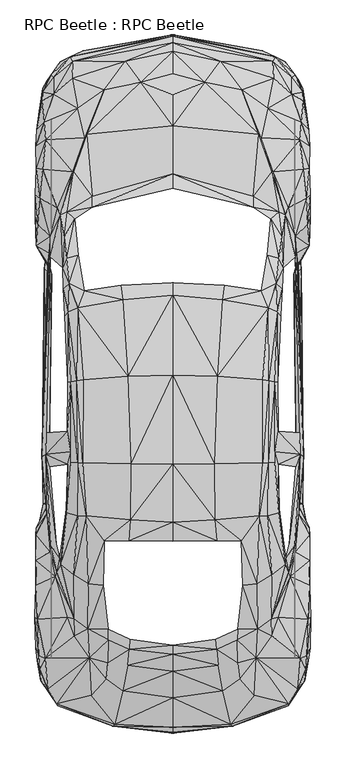
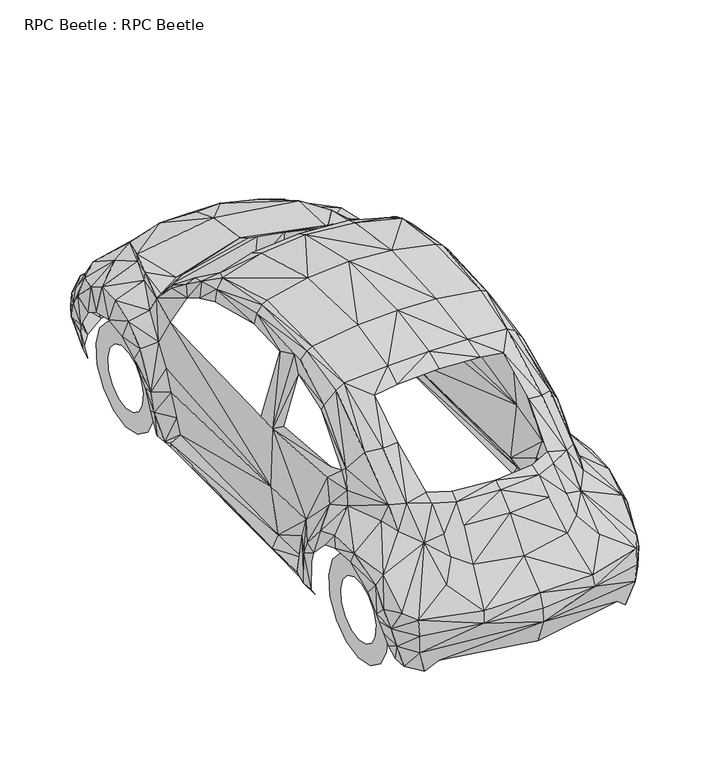
"""IFC4 building model written with IfcOpenShell, lengths in millimetres: proxy geometry, RPC Beetle : RPC Beetle."""

from ifc_helpers import new_model, si_unit, origin, place, context, project, spatial, triangles, source, transform, mapped, element, save


def rpc_beetle_rpc_beetle_e6dad58a(model_context):
    return source(origin(), model_context, "Body", "Tessellation", [
        triangles([(0.0, -748.5645555, 521.3897593), (0.0, -720.145796, 603.6245653), (0.0, -696.6751356, 283.1364967), (0.0, -552.6985313, 738.4055826), (0.0, -753.24988, 438.4543419), (0.0, -253.6668202, 1039.7142986), (0.0, -401.1027337, 921.397756), (0.0, -304.8118089, 1012.2589251), (0.0, 339.3171518, 1395.7149525), (0.0, 448.6132421, 1442.130724), (0.0, 778.0780157, 1504.0475842), (0.0, 1285.0174942, 1509.4774853), (0.0, 1741.0748314, 1402.3269035), (0.0, 2430.9628086, 967.2005562), (0.0, 3130.0025528, 632.0433249), (0.0, 3001.4394699, 771.5097393), (0.0, 2704.2468544, 928.754211), (0.0, 3164.2013374, 220.1686106), (0.0, 2883.1667473, 858.7363918), (0.0, 3222.5277191, 395.8043289), (0.0, 3179.0018875, 555.7637512), (0.0, 3213.9451035, 530.2788242), (-338.1786312, -715.5042189, 523.0099365), (-331.0411308, -702.1487114, 593.4656287), (-244.7339716, -218.0229748, 1034.0655882), (-248.9814594, -275.9551764, 1002.9319508), (-257.7391552, -368.1737844, 911.8518997), (-249.0690268, 342.8202084, 1381.001897), (-285.2383307, -511.5373446, 760.4312004), (-240.1361781, 460.085834, 1426.5857426), (-236.4579324, 780.8804609, 1493.4070999), (-652.4925127, -590.2252742, 370.4945729), (-540.0874552, -593.3342777, 283.4430006), (-181.240627, 2954.2792671, 806.3215679), (-253.1851454, 1278.5806778, 1496.1656525), (-379.8652946, -444.3657907, 798.2645016), (-370.9324459, -353.3294506, 889.169418), (-367.9986134, -222.226679, 1003.4574274), (-368.3927027, -160.7038173, 1036.6928988), (-390.1556185, 342.8640284, 1359.0200993), (-282.5672364, 1713.2691158, 1399.3055763), (-397.3369025, 87.4894363, 1215.350017), (-463.1072702, -537.7666666, 704.819842), (-271.488752, 3072.3331078, 662.6953056), (-475.7621301, -323.0715955, 849.8473269), (-463.7202779, 3085.9075699, 214.2571618), (-482.2428391, 95.7654664, 1203.3957321), (-485.0452844, -159.3025947, 1005.0776047), (-568.725133, 3071.5011818, 546.7432989), (-493.54026, 483.2499724, 1391.2922573), (-583.2629085, 3099.3942467, 522.0465869), (-510.267473, 3132.2794487, 369.399836), (-391.8633631, 2911.6292542, 782.7633402), (-656.3459112, -597.8445039, 480.0971852), (-660.2431297, -584.8393021, 576.2567591), (-562.2882076, -200.069692, 879.711129), (-560.0550227, -101.4579695, 987.1680874), (-512.4569106, 786.1788294, 1448.4362984), (-541.7951998, 484.7825824, 1359.8520252), (-563.9959886, 148.5744068, 1172.3059147), (-608.4850971, -561.2372907, 218.460866), (-511.2746063, 1258.5255066, 1456.1868427), (-542.4082438, 784.6900394, 1430.6581684), (-458.8597824, 2304.063723, 949.0283369), (-601.0410384, -92.7440574, 893.1979511), (-503.7429803, 1765.2899231, 1320.9679161), (-546.0426876, 1253.0081108, 1441.51768), (-603.0115213, 501.1594534, 1278.5806778), (-580.1539412, 788.8937799, 1378.7250011), (-607.2152255, 519.8571493, 1235.1424862), (-601.2599931, 965.2738569, 1337.0383015), (-712.482819, -503.0861526, 590.4880125), (-542.6709821, 1670.0499516, 1361.1657532), (-490.6064275, 2657.8746849, 893.5044731), (-599.6398158, 778.0780157, 1307.3059593), (-598.0634222, 1243.7249565, 1343.7817852), (-639.5749146, 208.1267766, 1062.4843477), (-680.4296156, -470.200987, 218.6798025), (-538.4672779, 1966.7170177, 1180.5819357), (-580.9859035, 1248.2351463, 1401.7577522), (-644.5230137, 243.2889472, 1028.2854904), (-502.3417577, 2635.8053925, 866.0052795), (-660.7247864, 162.2364272, 955.2462713), (-690.2382465, -396.5925076, 226.8244725), (-559.1354568, 2175.0189835, 1011.1642244), (-670.1830753, 140.867628, 872.7049433), (-662.476351, 324.2976834, 1009.4564798), (-615.0971935, 1623.4589001, 1262.1161304), (-594.647933, 1646.0976345, 1321.2744381), (-589.4370955, 1809.603788, 1269.4287655), (-728.8159063, -481.9801008, 373.2094508), (-751.5859554, -454.4371236, 476.5503087), (-694.0478251, 315.3210511, 957.7860146), (-726.5826851, -327.3190833, 735.5593174), (-622.9353052, 1777.2441353, 1192.7989225), (-564.6528162, 2445.7196114, 934.1402195), (-731.7935589, -393.8776297, 324.1225488), (-571.0021379, 2444.2743507, 884.1775715), (-698.6456549, 279.8523585, 807.6352232), (-604.281393, 1949.7708138, 1170.4667828), (-587.422829, 3013.0873055, 200.1134757), (-690.9388578, 574.2424925, 283.6181534), (-750.2284801, -381.0038152, 396.9865969), (-627.533135, 1896.2612892, 1124.7078026), (-602.486081, 2215.5670898, 949.1596516), (-619.4322487, 2072.8166462, 1075.2705585), (-710.4685524, 549.6333478, 448.6132421), (-764.7225082, -360.3356363, 467.5298927), (-699.5214008, 762.6206743, 1015.4992796), (-763.3212856, -313.2191809, 670.9275066), (-757.8477098, -390.9437971, 564.6528162), (-717.4746655, 496.2989579, 583.5694304), (-722.7292866, 461.2243546, 180.9779068), (-717.6498728, 554.4500959, 179.883188), (-771.4659193, -341.8130751, 511.011868), (-573.9359705, 2975.4727409, 682.6190168), (-730.7864256, 375.880545, 185.1815928), (-541.1821558, 2805.3982384, 782.9385475), (-639.7501219, 2198.4457512, 944.2553724), (-738.9310593, 551.5600471, 222.4018318), (-781.5810722, -268.773856, 609.2294921), (-772.2979179, -106.055763, 755.9210106), (-721.7221533, 957.7422672, 967.0254215), (-703.3309793, 810.1311464, 292.3320837), (-724.8311932, 835.0468494, 964.354291), (-757.7601425, 370.5383566, 225.4670335), (-785.3469034, -89.941594, 695.4928677), (-779.654373, 80.9211599, 675.5690838), (-779.391671, 89.5037119, 754.6511026), (-760.3874531, 444.1030523, 223.1462268), (-778.0780157, 192.1001749, 630.9048042), (-658.6229525, 2237.154871, 849.7597595), (-770.9404427, 345.4913389, 426.193535), (-774.1807972, 315.1458801, 501.68493), (-781.1869829, 232.2542464, 695.886957), (-719.22623, 810.0873991, 185.8384204), (-689.8879045, 1858.8658974, 293.9084591), (-696.6751356, 1958.8788334, 956.4286119), (-779.7419403, 377.3693713, 532.3806581), (-778.121763, 416.9979481, 439.7241772), (-745.4993357, 819.5895081, 613.6521509), (-677.7147377, 2884.8305992, 670.6209846), (-697.5509542, 2077.4143307, 756.8843239), (-639.6187346, 3069.1803932, 391.6881921), (-713.0082956, 1918.243087, 536.7157496), (-718.1752768, 1909.8794987, 192.9759572), (-705.1701113, 1981.9554771, 648.2888449), (-730.7864256, 1891.0943081, 233.348947), (-673.9927265, 2907.8634956, 198.6684513), (-726.8892071, 2038.9242382, 189.9545391), (-721.634586, 1973.3728615, 189.9545391), (-678.1963943, 2982.566494, 540.5253282), (-699.6089682, 2815.6885986, 206.2000773), (-696.3686136, 2991.5871643, 517.4050097), (-723.6488525, 2624.6831062, 787.5801247), (-699.0834915, 1882.4679451, 390.3745368), (-764.8976429, 2042.1645927, 362.5688576), (-741.7773245, 2457.6738235, 808.6861765), (-716.1610102, 2965.1387787, 449.5328081), (-766.4302528, 2001.1348297, 376.5811563), (-731.5746042, 2724.4334129, 727.6336384), (-771.1593973, 2084.5957237, 482.2428391), (-759.1175451, 2291.4088268, 780.0922823), (-769.0137434, 2143.3161221, 699.0397442), (-777.5525391, 2022.8538528, 494.8101316), (-742.4779358, 2846.8660561, 601.8730371), (-782.1065489, 2185.659613, 616.4545961), (-739.5441032, 2918.4163399, 427.3758393), (-741.1204605, 2896.5223274, 519.8133657), (-750.4036148, 2804.4349251, 398.0813338), (-782.2378635, 2313.1717426, 680.7361376), (-778.0780157, 2462.7970573, 693.5223484), (-759.9057238, 2786.6130478, 455.2253386), (-774.1807972, 2682.8342079, 602.6612157), (-780.3549843, 2589.4335136, 666.3297495), (-742.6093231, 809.1240131, 220.3875652), (0.0, 2349.0782719, 1011.1642244), (-458.8597824, 2239.9573162, 1006.6102146), (0.0, 1812.0122166, 1368.2157589), (-293.9522428, 1795.8104439, 1359.1514866), (-580.2415086, 849.7160122, 1381.7900757), (338.1786312, -715.5042189, 523.0099365), (331.0411308, -702.1487114, 593.4656287), (244.7339716, -218.0229748, 1034.0655882), (248.9814594, -275.9551764, 1002.9319508), (257.7391552, -368.1737844, 911.8518997), (249.0690268, 342.8202084, 1381.001897), (285.2383307, -511.5373446, 760.4312004), (240.1361781, 460.085834, 1426.5857426), (236.4579324, 780.8804609, 1493.4070999), (652.4925127, -590.2252742, 370.4945729), (540.0874552, -593.3342777, 283.4430006), (181.240627, 2954.2792671, 806.3215679), (253.1851454, 1278.5806778, 1496.1656525), (379.8652946, -444.3657907, 798.2645016), (370.9324459, -353.3294506, 889.169418), (367.9986134, -222.226679, 1003.4574274), (368.3927027, -160.7038173, 1036.6928988), (390.1556185, 342.8640284, 1359.0200993), (282.5672364, 1713.2691158, 1399.3055763), (397.3369025, 87.4894363, 1215.350017), (463.1072702, -537.7666666, 704.819842), (271.488752, 3072.3331078, 662.6953056), (475.7621301, -323.0715955, 849.8473269), (463.7202779, 3085.9075699, 214.2571618), (482.2428391, 95.7654664, 1203.3957321), (485.0452844, -159.3025947, 1005.0776047), (568.725133, 3071.5011818, 546.7432989), (493.54026, 483.2499724, 1391.2922573), (583.2629085, 3099.3942467, 522.0465869), (510.267473, 3132.2794487, 369.399836), (391.8633631, 2911.6292542, 782.7633402), (656.3459112, -597.8445039, 480.0971852), (660.2431297, -584.8393021, 576.2567591), (562.2882076, -200.069692, 879.711129), (560.0550227, -101.4579695, 987.1680874), (512.4569106, 786.1788294, 1448.4362984), (541.7951998, 484.7825824, 1359.8520252), (563.9959886, 148.5744068, 1172.3059147), (608.4850971, -561.2372907, 218.460866), (511.2746063, 1258.5255066, 1456.1868427), (542.4082438, 784.6900394, 1430.6581684), (458.8597824, 2304.063723, 949.0283369), (601.0410384, -92.7440574, 893.1979511), (503.7429803, 1765.2899231, 1320.9679161), (546.0426876, 1253.0081108, 1441.51768), (603.0115213, 501.1594534, 1278.5806778), (580.1539412, 788.8937799, 1378.7250011), (607.2152255, 519.8571493, 1235.1424862), (601.2599931, 965.2738569, 1337.0383015), (712.482819, -503.0861526, 590.4880125), (542.6709821, 1670.0499516, 1361.1657532), (490.6064275, 2657.8746849, 893.5044731), (599.6398158, 778.0780157, 1307.3059593), (598.0634222, 1243.7249565, 1343.7817852), (639.5749146, 208.1267766, 1062.4843477), (680.4734356, -470.200987, 218.6798025), (538.4672779, 1966.7170177, 1180.5819357), (580.9859035, 1248.2351463, 1401.7577522), (644.5230137, 243.2889472, 1028.2854904), (502.3417577, 2635.8053925, 866.0052795), (660.7247864, 162.2364272, 955.2462713), (690.2382465, -396.5925076, 226.8244725), (559.1354568, 2175.0189835, 1011.1642244), (670.1830753, 140.867628, 872.7049433), (662.476351, 324.2976834, 1009.4564798), (615.0971935, 1623.4589001, 1262.1161304), (594.647933, 1646.0976345, 1321.2744381), (589.4370955, 1809.603788, 1269.4287655), (728.8159063, -481.9801008, 373.2094508), (751.5859554, -454.4371236, 476.5503087), (694.0478251, 315.3210511, 957.7860146), (726.5826851, -327.3190833, 735.5593174), (622.9353052, 1777.2441353, 1192.7989225), (564.6528162, 2445.7196114, 934.1402195), (731.7935589, -393.8776297, 324.1225488), (571.0021379, 2444.2743507, 884.1775715), (698.6456549, 279.8523585, 807.6352232), (604.281393, 1949.7708138, 1170.4667828), (587.422829, 3013.0873055, 200.1134757), (690.9388578, 574.2424925, 283.6181534), (750.2284801, -381.0038152, 396.9865969), (627.533135, 1896.2612892, 1124.7078026), (602.486081, 2215.5670898, 949.1596516), (619.4322487, 2072.8166462, 1075.2705585), (710.4685524, 549.6333478, 448.6132421), (764.7225082, -360.3356363, 467.5298927), (699.5214008, 762.6206743, 1015.4992796), (763.3212856, -313.2191809, 670.9275066), (757.8477098, -390.9437971, 564.6528162), (717.4746655, 496.2989579, 583.5694304), (722.7292866, 461.2243546, 180.9779068), (717.6498728, 554.4500959, 179.883188), (771.4659193, -341.8130751, 511.011868), (573.9359705, 2975.4727409, 682.6190168), (730.7864256, 375.880545, 185.1815928), (541.1821558, 2805.3982384, 782.9385475), (639.7501219, 2198.4457512, 944.2553724), (738.9310593, 551.5600471, 222.4018318), (781.5810722, -268.773856, 609.2294921), (772.2979179, -106.055763, 755.9210106), (721.7659733, 957.7422672, 967.0254215), (703.3309793, 810.1311464, 292.3320837), (724.8311932, 835.0468494, 964.354291), (757.7601425, 370.5383566, 225.4670335), (785.3469034, -89.941594, 695.4928677), (779.654373, 80.9211599, 675.5690838), (779.4354183, 89.5037119, 754.6511026), (760.3874531, 444.1030523, 223.1462268), (778.0780157, 192.1001749, 630.9048042), (658.6229525, 2237.154871, 849.7597595), (770.9404427, 345.4913389, 426.193535), (774.1807972, 315.1458801, 501.68493), (781.1869829, 232.2542464, 695.886957), (719.22623, 810.0873991, 185.8384204), (689.8879045, 1858.8658974, 293.9084591), (696.6751356, 1958.8788334, 956.4286119), (779.7419403, 377.3693713, 532.3806581), (778.121763, 416.9979481, 439.7241772), (745.4993357, 819.5895081, 613.6521509), (677.7147377, 2884.8305992, 670.6209846), (697.5509542, 2077.4143307, 756.8843239), (639.6187346, 3069.1803932, 391.6881921), (713.0082956, 1918.243087, 536.7157496), (718.1752768, 1909.8794987, 192.9759572), (705.1701113, 1981.9554771, 648.2888449), (730.7864256, 1891.0943081, 233.348947), (673.9927265, 2907.8634956, 198.6684513), (726.8892071, 2038.9242382, 189.9545391), (721.634586, 1973.3728615, 189.9545391), (678.1963943, 2982.566494, 540.5253282), (699.6089682, 2815.6885986, 206.2000773), (696.3686136, 2991.5871643, 517.4050097), (723.6488525, 2624.6831062, 787.5801247), (699.0834915, 1882.4679451, 390.3745368), (764.8976429, 2042.1645927, 362.5688576), (741.7773245, 2457.6738235, 808.6861765), (716.1610102, 2965.1387787, 449.5328081), (766.4302528, 2001.1348297, 376.5811563), (731.5746042, 2724.4334129, 727.6336384), (771.2032173, 2084.5957237, 482.2428391), (759.1175451, 2291.4088268, 780.0922823), (769.0137434, 2143.3161221, 699.0397442), (777.5525391, 2022.8538528, 494.8101316), (742.4779358, 2846.8660561, 601.8730371), (782.1065489, 2185.659613, 616.4545961), (739.5441032, 2918.4163399, 427.3758393), (741.1204605, 2896.5223274, 519.8133657), (750.4036148, 2804.4349251, 398.0813338), (782.2378635, 2313.1717426, 680.7361376), (778.0780157, 2462.7970573, 693.5223484), (759.9057238, 2786.6130478, 455.2253386), (774.1807972, 2682.8342079, 602.6612157), (780.3549843, 2589.4335136, 666.3297495), (742.6093231, 809.1240131, 220.3875652), (458.8597824, 2239.9573162, 1006.6102146), (293.9522428, 1795.8104439, 1359.1514866), (580.2415086, 849.7160122, 1381.7900757), (-693.1720791, 2430.2621246, 0.0015107), (-693.1720791, 2430.2621246, 117.8363848), (-693.1720791, 2557.1174629, 26.9752316), (-693.1720791, 2507.7678589, 134.3008595), (-693.1720791, 2661.9910034, 103.1672311), (-693.1720791, 2571.918013, 180.8918292), (-693.1720791, 2726.8416962, 215.4847577), (-693.1720791, 2611.5466988, 249.5522095), (-693.1720791, 2740.4161583, 344.4419117), (-693.1720791, 2619.8226471, 328.3715263), (-693.1720791, 2700.3497086, 467.7941208), (-693.1720791, 2595.3447807, 403.731534), (-693.1720791, 2613.56082, 564.1288656), (-693.1720791, 2542.3169128, 462.6271033), (-693.1720791, 2495.1128174, 616.8940315), (-693.1720791, 2469.8908104, 494.899225), (-693.1720791, 2365.4114319, 616.8940315), (-693.1720791, 2390.6335842, 494.899225), (-693.1720791, 2246.9634293, 564.1288656), (-693.1720791, 2318.2073364, 462.6271033), (-693.1720791, 2160.1746861, 467.7941208), (-693.1720791, 2265.1794685, 403.731534), (-693.1720791, 2120.108091, 344.4419117), (-693.1720791, 2240.7017475, 328.3715263), (-693.1720791, 2133.6825531, 215.4847577), (-693.1720791, 2248.9776958, 249.5522095), (-693.1720791, 2198.5333912, 103.1672311), (-693.1720791, 2288.6063816, 180.8918292), (-693.1720791, 2303.4067863, 26.9752316), (-693.1720791, 2352.7565357, 134.3008595), (693.1720791, 2430.2621246, 0.0015107), (693.1720791, 2430.2621246, 117.8363848), (693.1720791, 2303.4067863, 26.9752316), (693.1720791, 2352.7565357, 134.3008595), (693.1720791, 2198.5333912, 103.1672311), (693.1720791, 2288.6063816, 180.8918292), (693.1720791, 2133.6825531, 215.4847577), (693.1720791, 2248.9776958, 249.5522095), (693.1720791, 2120.108091, 344.4419117), (693.1720791, 2240.7017475, 328.3715263), (693.1720791, 2160.1746861, 467.7941208), (693.1720791, 2265.1794685, 403.731534), (693.1720791, 2246.9634293, 564.1288656), (693.1720791, 2318.2073364, 462.6271033), (693.1720791, 2365.4114319, 616.8940315), (693.1720791, 2390.6335842, 494.899225), (693.1720791, 2495.1128174, 616.8940315), (693.1720791, 2469.8908104, 494.899225), (693.1720791, 2613.56082, 564.1288656), (693.1720791, 2542.3169128, 462.6271033), (693.1720791, 2700.3497086, 467.7941208), (693.1720791, 2595.3447807, 403.731534), (693.1720791, 2740.4161583, 344.4419117), (693.1720791, 2619.8226471, 328.3715263), (693.1720791, 2726.8416962, 215.4847577), (693.1720791, 2611.5466988, 249.5522095), (693.1720791, 2661.9910034, 103.1672311), (693.1720791, 2571.918013, 180.8918292), (693.1720791, 2557.1174629, 26.9752316), (693.1720791, 2507.7678589, 134.3008595), (-693.1720791, -13.5744371, 0.0015107), (-693.1720791, -13.5744371, 117.8363848), (-693.1720791, 113.2808671, 26.9752316), (-693.1720791, 63.9312222, 134.3008595), (-693.1720791, 218.154344, 103.1672311), (-693.1720791, 128.0813808, 180.8918292), (-693.1720791, 283.0051276, 215.4847577), (-693.1720791, 167.7099848, 249.5522095), (-693.1720791, 296.5795534, 344.4419117), (-693.1720791, 175.9860058, 328.3715263), (-693.1720791, 256.5130673, 467.7941208), (-693.1720791, 151.5082394, 403.731534), (-693.1720791, 169.7242514, 564.1288656), (-693.1720791, 98.4803533, 462.6271033), (-693.1720791, 51.2763442, 616.8940315), (-693.1720791, 26.0541623, 494.899225), (-693.1720791, -78.4252185, 616.8940315), (-693.1720791, -53.2030343, 494.899225), (-693.1720791, -196.8731212, 564.1288656), (-693.1720791, -125.6292322, 462.6271033), (-693.1720791, -283.6619552, 467.7941208), (-693.1720791, -178.6571182, 403.731534), (-693.1720791, -323.7284231, 344.4419117), (-693.1720791, -203.1348938, 328.3715263), (-693.1720791, -310.1539973, 215.4847577), (-693.1720791, -194.8588546, 249.5522095), (-693.1720791, -245.3032137, 103.1672311), (-693.1720791, -155.2302597, 180.8918292), (-693.1720791, -140.4297459, 26.9752316), (-693.1720791, -91.0800965, 134.3008595), (693.1720791, -13.5744371, 0.0015107), (693.1720791, -13.5744371, 117.8363848), (693.1720791, -140.4297459, 26.9752316), (693.1720791, -91.0800965, 134.3008595), (693.1720791, -245.3032137, 103.1672311), (693.1720791, -155.2302597, 180.8918292), (693.1720791, -310.1539973, 215.4847577), (693.1720791, -194.8588546, 249.5522095), (693.1720791, -323.7284231, 344.4419117), (693.1720791, -203.1348938, 328.3715263), (693.1720791, -283.6619552, 467.7941208), (693.1720791, -178.6571182, 403.731534), (693.1720791, -196.8731212, 564.1288656), (693.1720791, -125.6292322, 462.6271033), (693.1720791, -78.4252185, 616.8940315), (693.1720791, -53.2030343, 494.899225), (693.1720791, 51.2763442, 616.8940315), (693.1720791, 26.0541623, 494.899225), (693.1720791, 169.7242514, 564.1288656), (693.1720791, 98.4803533, 462.6271033), (693.1720791, 256.5130673, 467.7941208), (693.1720791, 151.5082394, 403.731534), (693.1720791, 296.5795534, 344.4419117), (693.1720791, 175.9860058, 328.3715263), (693.1720791, 283.0051276, 215.4847577), (693.1720791, 167.7099848, 249.5522095), (693.1720791, 218.154344, 103.1672311), (693.1720791, 128.0813808, 180.8918292), (693.1720791, 113.2808671, 26.9752316), (693.1720791, 63.9312222, 134.3008595)], [[67, 58, 62], [67, 63, 58], [53, 82, 74], [34, 17, 19], [118, 82, 53], [155, 98, 82], [155, 158, 98], [34, 74, 17], [172, 155, 175], [172, 158, 155], [159, 168, 169], [166, 142, 169], [175, 161, 174], [175, 155, 161], [142, 152, 169], [154, 169, 152], [160, 145, 165], [160, 156, 145], [162, 160, 165], [162, 157, 160], [34, 53, 74], [74, 96, 64], [82, 96, 74], [82, 98, 96], [36, 29, 27], [29, 43, 24], [23, 55, 54], [23, 24, 55], [23, 2, 24], [23, 1, 2], [5, 1, 23], [134, 140, 133], [134, 139, 140], [117, 130, 113], [117, 126, 130], [113, 120, 114], [113, 130, 120], [140, 112, 107], [140, 139, 112], [92, 108, 103], [91, 103, 97], [91, 92, 103], [61, 33, 32], [84, 78, 91], [84, 91, 97], [38, 26, 25], [77, 81, 83], [63, 50, 58], [63, 59, 50], [68, 63, 69], [68, 59, 63], [181, 75, 69], [74, 64, 17], [64, 14, 17], [64, 178, 14], [178, 177, 14], [34, 19, 16], [53, 34, 44], [21, 44, 15], [21, 49, 44], [44, 34, 15], [34, 16, 15], [22, 49, 21], [22, 51, 49], [20, 51, 22], [20, 52, 51], [18, 52, 20], [18, 46, 52], [51, 152, 49], [51, 154, 152], [101, 144, 46], [144, 52, 46], [101, 159, 144], [159, 169, 154], [101, 168, 159], [101, 149, 168], [149, 170, 168], [149, 153, 170], [168, 173, 169], [168, 170, 173], [49, 142, 116], [49, 152, 142], [49, 116, 44], [116, 142, 118], [161, 155, 118], [155, 82, 118], [142, 161, 118], [158, 132, 98], [158, 163, 132], [172, 163, 158], [172, 171, 163], [98, 119, 96], [98, 132, 119], [171, 164, 163], [171, 167, 164], [163, 143, 132], [163, 164, 143], [96, 105, 64], [96, 119, 105], [105, 178, 64], [105, 85, 178], [167, 165, 164], [167, 162, 165], [165, 143, 164], [165, 147, 143], [150, 160, 157], [150, 151, 160], [151, 156, 160], [151, 148, 137], [13, 35, 12], [13, 41, 35], [12, 31, 11], [12, 35, 31], [35, 58, 31], [35, 62, 58], [11, 30, 10], [11, 31, 30], [31, 50, 30], [31, 58, 50], [10, 28, 9], [10, 30, 28], [30, 40, 28], [30, 50, 40], [125, 75, 181], [125, 109, 75], [125, 87, 109], [125, 93, 87], [123, 141, 125], [137, 141, 156], [137, 124, 141], [148, 124, 137], [148, 176, 124], [146, 176, 148], [146, 136, 176], [141, 112, 125], [112, 93, 125], [112, 99, 93], [124, 112, 141], [124, 107, 112], [124, 102, 107], [176, 102, 124], [176, 120, 102], [136, 120, 176], [136, 114, 120], [47, 40, 50], [47, 42, 40], [48, 42, 47], [48, 39, 42], [57, 47, 60], [57, 48, 47], [60, 50, 59], [60, 47, 50], [59, 77, 60], [59, 68, 77], [77, 57, 60], [77, 83, 57], [70, 77, 68], [70, 81, 77], [75, 68, 69], [75, 70, 68], [26, 6, 25], [26, 8, 6], [27, 8, 26], [27, 7, 8], [29, 7, 27], [29, 4, 7], [24, 4, 29], [24, 2, 4], [32, 5, 23], [33, 5, 32], [33, 3, 5], [32, 23, 54], [55, 45, 72], [55, 24, 43], [99, 83, 93], [99, 86, 83], [135, 86, 99], [135, 129, 86], [131, 129, 135], [131, 128, 129], [93, 81, 87], [93, 83, 81], [128, 122, 129], [128, 127, 122], [122, 86, 129], [122, 65, 86], [86, 57, 83], [86, 65, 57], [127, 110, 122], [127, 121, 110], [110, 94, 122], [122, 94, 65], [94, 56, 65], [56, 57, 65], [56, 48, 57], [56, 45, 48], [94, 45, 56], [115, 110, 121], [115, 111, 110], [111, 94, 110], [111, 72, 94], [108, 92, 115], [92, 111, 115], [78, 32, 91], [78, 61, 32], [45, 38, 48], [45, 37, 38], [37, 26, 38], [37, 27, 26], [36, 27, 37], [134, 135, 139], [134, 131, 135], [139, 99, 112], [139, 135, 99], [126, 140, 130], [126, 133, 140], [130, 107, 120], [130, 140, 107], [120, 107, 102], [45, 36, 37], [92, 55, 72], [92, 54, 55], [91, 54, 92], [91, 32, 54], [92, 72, 111], [72, 45, 94], [43, 45, 55], [43, 36, 45], [43, 29, 36], [79, 90, 66], [79, 100, 90], [90, 73, 66], [85, 100, 79], [85, 106, 100], [85, 105, 106], [105, 119, 106], [95, 88, 89], [90, 89, 73], [89, 67, 73], [73, 67, 62], [89, 76, 80], [89, 80, 67], [88, 76, 89], [73, 35, 41], [73, 62, 35], [69, 63, 181], [80, 63, 67], [76, 71, 80], [146, 148, 151], [141, 147, 145], [151, 137, 156], [173, 166, 169], [173, 174, 166], [166, 174, 161], [166, 161, 142], [52, 144, 51], [144, 154, 51], [144, 159, 154], [116, 53, 44], [116, 118, 53], [119, 143, 138], [143, 119, 132], [143, 147, 138], [138, 104, 119], [119, 104, 106], [104, 100, 106], [104, 90, 100], [104, 95, 90], [95, 89, 90], [25, 39, 38], [38, 39, 48], [141, 138, 147], [156, 141, 145], [165, 145, 147], [41, 179, 180], [41, 13, 179], [66, 41, 180], [66, 73, 41], [123, 125, 71], [125, 181, 71], [71, 181, 80], [181, 63, 80], [138, 141, 123], [226, 221, 217], [226, 217, 222], [212, 233, 241], [193, 19, 17], [277, 212, 241], [314, 241, 257], [314, 257, 317], [193, 17, 233], [331, 334, 314], [331, 314, 317], [318, 328, 327], [325, 328, 301], [334, 333, 320], [334, 320, 314], [301, 328, 311], [313, 311, 328], [319, 324, 304], [319, 304, 315], [321, 324, 319], [321, 319, 316], [193, 233, 212], [233, 223, 255], [241, 233, 255], [241, 255, 257], [195, 186, 188], [188, 183, 202], [182, 213, 214], [182, 214, 183], [182, 183, 2], [182, 2, 1], [5, 182, 1], [293, 292, 299], [293, 299, 298], [276, 272, 289], [276, 289, 285], [272, 273, 279], [272, 279, 289], [299, 266, 271], [299, 271, 298], [251, 262, 267], [250, 256, 262], [250, 262, 251], [220, 191, 192], [243, 250, 237], [243, 256, 250], [197, 184, 185], [236, 242, 240], [222, 217, 209], [222, 209, 218], [227, 228, 222], [227, 222, 218], [338, 228, 234], [233, 17, 223], [223, 17, 14], [223, 14, 336], [336, 14, 177], [193, 16, 19], [212, 203, 193], [21, 15, 203], [21, 203, 208], [203, 15, 193], [193, 15, 16], [22, 21, 208], [22, 208, 210], [20, 22, 210], [20, 210, 211], [18, 20, 211], [18, 211, 205], [210, 208, 311], [210, 311, 313], [260, 205, 303], [303, 205, 211], [260, 303, 318], [318, 313, 328], [260, 318, 327], [260, 327, 308], [308, 327, 329], [308, 329, 312], [327, 328, 332], [327, 332, 329], [208, 275, 301], [208, 301, 311], [208, 203, 275], [275, 277, 301], [320, 277, 314], [314, 277, 241], [301, 277, 320], [317, 257, 291], [317, 291, 322], [331, 317, 322], [331, 322, 330], [257, 255, 278], [257, 278, 291], [330, 322, 323], [330, 323, 326], [322, 291, 302], [322, 302, 323], [255, 223, 264], [255, 264, 278], [264, 223, 336], [264, 336, 244], [326, 323, 324], [326, 324, 321], [324, 323, 302], [324, 302, 306], [309, 316, 319], [309, 319, 310], [310, 319, 315], [310, 296, 307], [13, 12, 194], [13, 194, 200], [12, 11, 190], [12, 190, 194], [194, 190, 217], [194, 217, 221], [11, 10, 189], [11, 189, 190], [190, 189, 209], [190, 209, 217], [10, 9, 187], [10, 187, 189], [189, 187, 199], [189, 199, 209], [284, 338, 234], [284, 234, 268], [284, 268, 246], [284, 246, 252], [282, 284, 300], [296, 315, 300], [296, 300, 283], [307, 296, 283], [307, 283, 335], [305, 307, 335], [305, 335, 295], [300, 284, 271], [271, 284, 252], [271, 252, 258], [283, 300, 271], [283, 271, 266], [283, 266, 261], [335, 283, 261], [335, 261, 279], [295, 335, 279], [295, 279, 273], [206, 209, 199], [206, 199, 201], [207, 206, 201], [207, 201, 198], [216, 219, 206], [216, 206, 207], [219, 218, 209], [219, 209, 206], [218, 219, 236], [218, 236, 227], [236, 219, 216], [236, 216, 242], [229, 227, 236], [229, 236, 240], [234, 228, 227], [234, 227, 229], [185, 184, 6], [185, 6, 8], [186, 185, 8], [186, 8, 7], [188, 186, 7], [188, 7, 4], [183, 188, 4], [183, 4, 2], [191, 182, 5], [192, 191, 5], [192, 5, 3], [191, 213, 182], [214, 231, 204], [214, 202, 183], [258, 252, 242], [258, 242, 245], [294, 258, 245], [294, 245, 288], [290, 294, 288], [290, 288, 287], [252, 246, 240], [252, 240, 242], [287, 288, 281], [287, 281, 286], [281, 288, 245], [281, 245, 224], [245, 242, 216], [245, 216, 224], [286, 281, 269], [286, 269, 280], [269, 281, 253], [281, 224, 253], [253, 224, 215], [215, 224, 216], [215, 216, 207], [215, 207, 204], [253, 215, 204], [274, 280, 269], [274, 269, 270], [270, 269, 253], [270, 253, 231], [267, 274, 251], [251, 274, 270], [237, 250, 191], [237, 191, 220], [204, 207, 197], [204, 197, 196], [196, 197, 185], [196, 185, 186], [195, 196, 186], [293, 298, 294], [293, 294, 290], [298, 271, 258], [298, 258, 294], [285, 289, 299], [285, 299, 292], [289, 279, 266], [289, 266, 299], [279, 261, 266], [204, 196, 195], [251, 231, 214], [251, 214, 213], [250, 251, 213], [250, 213, 191], [251, 270, 231], [231, 253, 204], [202, 214, 204], [202, 204, 195], [202, 195, 188], [238, 225, 249], [238, 249, 259], [249, 225, 232], [244, 238, 259], [244, 259, 265], [244, 265, 264], [264, 265, 278], [254, 248, 247], [249, 232, 248], [248, 232, 226], [232, 221, 226], [248, 239, 235], [248, 226, 239], [247, 248, 235], [232, 200, 194], [232, 194, 221], [228, 338, 222], [239, 226, 222], [235, 239, 230], [305, 310, 307], [300, 304, 306], [310, 315, 296], [332, 328, 325], [332, 325, 333], [325, 320, 333], [325, 301, 320], [211, 210, 303], [303, 210, 313], [303, 313, 318], [275, 203, 212], [275, 212, 277], [278, 297, 302], [302, 291, 278], [302, 297, 306], [297, 278, 263], [278, 265, 263], [263, 265, 259], [263, 259, 249], [263, 249, 254], [254, 249, 248], [184, 197, 198], [197, 207, 198], [300, 306, 297], [315, 304, 300], [324, 306, 304], [200, 337, 179], [200, 179, 13], [225, 337, 200], [225, 200, 232], [282, 230, 284], [284, 230, 338], [230, 239, 338], [338, 239, 222], [297, 282, 300], [339, 342, 341], [339, 340, 342], [341, 344, 343], [341, 342, 344], [343, 346, 345], [343, 344, 346], [345, 348, 347], [345, 346, 348], [347, 350, 349], [347, 348, 350], [349, 352, 351], [349, 350, 352], [351, 354, 353], [351, 352, 354], [353, 356, 355], [353, 354, 356], [355, 358, 357], [355, 356, 358], [357, 360, 359], [357, 358, 360], [359, 362, 361], [359, 360, 362], [361, 364, 363], [361, 362, 364], [363, 366, 365], [363, 364, 366], [365, 368, 367], [365, 366, 368], [367, 340, 339], [367, 368, 340], [369, 372, 371], [369, 370, 372], [371, 374, 373], [371, 372, 374], [373, 376, 375], [373, 374, 376], [375, 378, 377], [375, 376, 378], [377, 380, 379], [377, 378, 380], [379, 382, 381], [379, 380, 382], [381, 384, 383], [381, 382, 384], [383, 386, 385], [383, 384, 386], [385, 388, 387], [385, 386, 388], [387, 390, 389], [387, 388, 390], [389, 392, 391], [389, 390, 392], [391, 394, 393], [391, 392, 394], [393, 396, 395], [393, 394, 396], [395, 398, 397], [395, 396, 398], [397, 370, 369], [397, 398, 370], [399, 402, 401], [399, 400, 402], [401, 404, 403], [401, 402, 404], [403, 406, 405], [403, 404, 406], [405, 408, 407], [405, 406, 408], [407, 410, 409], [407, 408, 410], [409, 412, 411], [409, 410, 412], [411, 414, 413], [411, 412, 414], [413, 416, 415], [413, 414, 416], [415, 418, 417], [415, 416, 418], [417, 420, 419], [417, 418, 420], [419, 422, 421], [419, 420, 422], [421, 424, 423], [421, 422, 424], [423, 426, 425], [423, 424, 426], [425, 428, 427], [425, 426, 428], [427, 400, 399], [427, 428, 400], [429, 432, 431], [429, 430, 432], [431, 434, 433], [431, 432, 434], [433, 436, 435], [433, 434, 436], [435, 438, 437], [435, 436, 438], [437, 440, 439], [437, 438, 440], [439, 442, 441], [439, 440, 442], [441, 444, 443], [441, 442, 444], [443, 446, 445], [443, 444, 446], [445, 448, 447], [445, 446, 448], [447, 450, 449], [447, 448, 450], [449, 452, 451], [449, 450, 452], [451, 454, 453], [451, 452, 454], [453, 456, 455], [453, 454, 456], [455, 458, 457], [455, 456, 458], [457, 430, 429], [457, 458, 430]], closed=False),
    ])


if __name__ == "__main__":
    model = new_model("IFC4")
    model_context = context("Model", 3, world=origin())
    ifc_project = project(units=[si_unit("LENGTHUNIT", "METRE", prefix="MILLI")], contexts=[model_context])
    site = spatial("IfcSite", under=ifc_project)
    building = spatial("IfcBuilding", under=site)
    placement = place(None, origin())
    rpc_beetle_rpc_beetle_shape = rpc_beetle_rpc_beetle_e6dad58a(model_context)
    element("IfcBuildingElementProxy", 1, Name="RPC Beetle : RPC Beetle", ObjectType="RPC Beetle : RPC Beetle", at=placement, inside=building, context=model_context, shape_type="MappedRepresentation", body=[
        mapped(rpc_beetle_rpc_beetle_shape, transform((0.0, 0.0, 0.0), x_axis=(1.0, 0.0, 0.0), y_axis=(0.0, 1.0, 0.0), z_axis=(0.0, 0.0, 1.0))),
    ])
    save(model, "model.ifc")

# Revit data of these elements
# Type "RPC Beetle : RPC Beetle"
#   built-in parameter 1005198 = "{2, 15},{39, RPC-16-0U6E-L4EG-ENH1-J3KF-SVEL-0TX4-C0},{1, 0},{1, 0},{2, 37},{1, 8},{5, Color},{1, 0},{1, 0},{3, 0.8},{3, 0.8},{3, 0.8},{1, 8},{7, BBoxMin},{1, 0},{1, 0},{1, 0},{1, 0},{1, 0},{1, 8},{7, BBoxMax},{1, 0},{1, 0},{1, 0},{1, 0},{1, 0},{2, 11},{9, RPCTypeId},{1, 0},{1, 0},{39, RPC-16-0U6E-L4EG-ENH1-J3KF-SVEL-0TX4-C0},{1, 6},{14, RPCPlantHeight},{1, 0},{1, 0},{7, 4.91667},{2, 11},{11, RPCFilePath},{1, 0},{1, 0},{92, C:\\RevitRender\\Version2015940\\2017\\assetlibrary_base.fbm\\RPCs\\ArchVision_Demo_VW_Beetle4.rpc},{2, 11},{20, AdvancedUIDefinition},{1, 0},{1, 0},{0, },{2, 11},{10, AssetLibID},{1, 0},{1, 0},{36, 4D3F6E72-3F99-4203-98E9-AF80B3C7A7A4},{2, 11},{10, BaseSchema},{1, 0},{1, 0},{9, RPCSchema},{2, 11},{12, ExchangeGUID},{1, 0},{1, 0},{0, },{1, 2},{6, Hidden},{1, 0},{1, 0},{1, 0},{2, 11},{12, LocalizedUID},{1, 0},{1, 0},{0, },{1, 4},{11, RPCCategory},{1, 0},{1, 0},{1, 0},{2, 11},{8, RPCImage},{1, 0},{1, 0},{0, },{1, 4},{13, SchemaVersion},{1, 0},{1, 0},{1, 5},{2, 11},{12, UIDefinition},{1, 0},{1, 0},{0, },{2, 11},{6, UIName},{1, 0},{1, 0},{39, RPC-16-0U6E-L4EG-ENH1-J3KF-SVEL-0TX4-C0},{2, 11},{11, VersionGUID},{1, 0},{1, 0},{9, RPCSchema},{2, 11},{9, assettype},{1, 0},{1, 0},{11, RPCGeometry},{2, 11},{11, description},{1, 0},{1, 0},{0, },{2, 11},{9, localname},{1, 0},{1, 0},{3, RPC},{2, 11},{9, localtype},{1, 0},{1, 0},{3, RPC},{1, 4},{8, revision},{1, 0},{1, 0},{1, 1},{2, 11},{9, thumbnail},{1, 0},{1, 0},{0, },{1, 4},{7, version},{1, 0},{1, 0},{1, 1},{2, 14},{6, Height},{1, 0},{1, 0},{7, 4.91667},{1, 2},{20, RPC_Cast Reflections},{1, 0},{1, 0},{1, 1},{1, 4},{16, RPC_Transparency},{1, 0},{1, 0},{2, 18},{1, 4},{11, RPC_Tinting},{1, 0},{1, 0},{2, 50},{1, 2},{15, RPC_Use Tinting},{1, 0},{1, 0},{1, 0},{1, 2},{17, RPC_License Plate},{1, 0},{1, 0},{1, 0},{2, 11},{25, RPC_License Plate Texture},{1, 0},{1, 0},{64, __RPC:/object data/textures/car/plate/textures/default/rgb/0/0/0},{2, 11},{27, RPC_i_License Plate Texture},{1, 0},{1, 0},{0, },{1, 2},{16, RPC_Custom Plate},{1, 0},{1, 0},{1, 0},{2, 11},{27, RPC_License Plate File Name},{1, 0},{1, 0},{0, },{2, 11},{7, keyword},{1, 0},{1, 0},{27, :Geometry:RPC:VW Beetle [4]},{2, 11},{8, category},{1, 0},{1, 0},{21, :Auto_Economy/Midsize},{21, assetlibrary_base.fbx},{1, 5},"
#   built-in parameter 1005195 = "RPC-16-0U6E-L4EG-ENH1-J3KF-SVEL-0TX4-C0"
#   Height = 0
